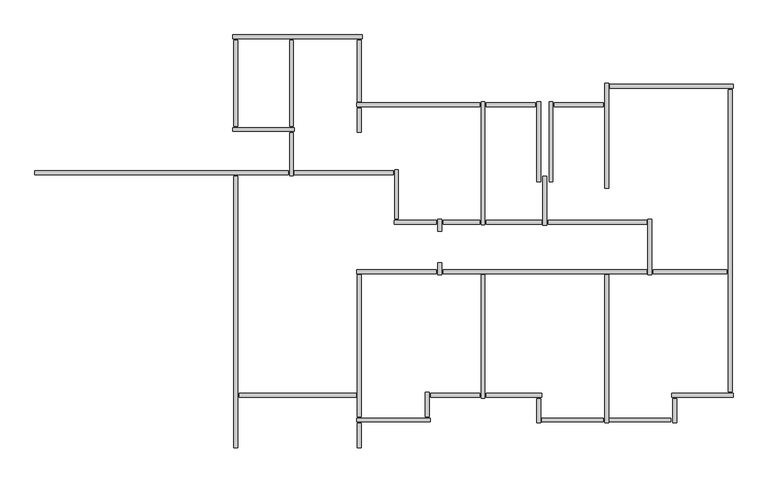
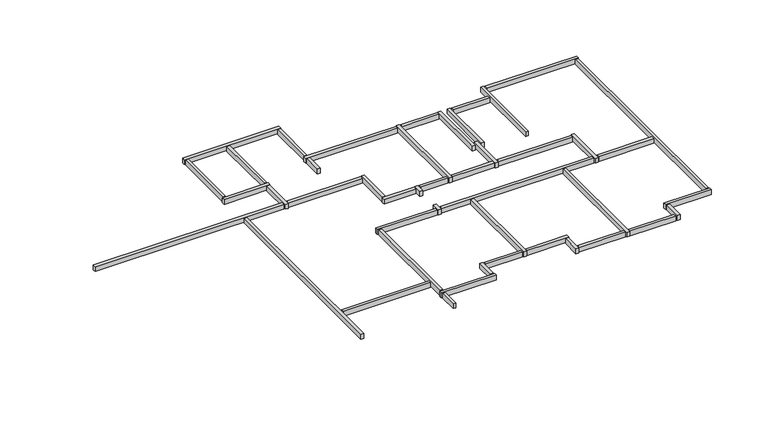
"""IFC4 building model written with IfcOpenShell, lengths in millimetres: beam geometry, Graute viga de respaldo8 : Graute viga de respaldo."""

from ifc_helpers import new_model, si_unit, frame, origin, place, context, project, spatial, polyline, outline, extrude, source, transform, mapped, element, save


def beam_c0cf02b6(model_context):
    return source(origin(), model_context, "Body", "SweptSolid", [
        extrude(outline(polyline([(-54994.9587292, 57408.4278788), (-54994.9587292, 57502.4278788), (-53804.9587292, 57502.4278788), (-53804.9587292, 57408.4278788), (-54994.9587292, 57408.4278788)])), frame((0.0, 0.0, 8632.9999999), z_axis=(0.0, 0.0, 1.0), x_axis=(1.0, 0.0, 0.0)), (0.0, 0.0, 1.0), 167.0),
        extrude(outline(polyline([(-56644.9587292, 57408.4278788), (-56644.9587292, 57502.4278788), (-55454.9587292, 57502.4278788), (-55454.9587292, 57408.4278788), (-56644.9587292, 57408.4278788)])), frame((0.0, 0.0, 8632.9999999), z_axis=(0.0, 0.0, 1.0), x_axis=(1.0, 0.0, 0.0)), (0.0, 0.0, 1.0), 167.0),
        extrude(outline(polyline([(-52594.9587292, 53358.4278788), (-52594.9587292, 53452.4278788), (-50804.9587292, 53452.4278788), (-50804.9587292, 53358.4278788), (-52594.9587292, 53358.4278788)])), frame((0.0, 0.0, 8632.9999999), z_axis=(0.0, 0.0, 1.0), x_axis=(1.0, 0.0, 0.0)), (0.0, 0.0, 1.0), 167.0),
        extrude(outline(polyline([(-57994.9587292, 50358.4278788), (-57994.9587292, 50452.4278788), (-56804.9587292, 50452.4278788), (-56804.9587292, 50358.4278788), (-57994.9587292, 50358.4278788)])), frame((0.0, 0.0, 8632.9999999), z_axis=(0.0, 0.0, 1.0), x_axis=(1.0, 0.0, 0.0)), (0.0, 0.0, 1.0), 167.0),
        extrude(outline(polyline([(-58121.9587292, 50475.4278788), (-58027.9587292, 50475.4278788), (-58027.9587292, 49885.4278788), (-58121.9587292, 49885.4278788), (-58121.9587292, 50475.4278788)])), frame((0.0, 0.0, 8632.9999999), z_axis=(0.0, 0.0, 1.0), x_axis=(1.0, 0.0, 0.0)), (0.0, 0.0, 1.0), 167.0),
        extrude(outline(polyline([(-59794.9587292, 49758.4278788), (-59794.9587292, 49852.4278788), (-58004.9587292, 49852.4278788), (-58004.9587292, 49758.4278788), (-59794.9587292, 49758.4278788)])), frame((0.0, 0.0, 8632.9999999), z_axis=(0.0, 0.0, 1.0), x_axis=(1.0, 0.0, 0.0)), (0.0, 0.0, 1.0), 167.0),
        extrude(outline(polyline([(-57727.9587292, 53335.4278788), (-57821.9587292, 53335.4278788), (-57821.9587292, 53625.4278788), (-57727.9587292, 53625.4278788), (-57727.9587292, 53335.4278788)])), frame((0.0, 0.0, 8632.9999999), z_axis=(0.0, 0.0, 1.0), x_axis=(1.0, 0.0, 0.0)), (0.0, 0.0, 1.0), 167.0),
        extrude(outline(polyline([(-55144.9587292, 54558.4278788), (-55144.9587292, 54652.4278788), (-52754.9587292, 54652.4278788), (-52754.9587292, 54558.4278788), (-55144.9587292, 54558.4278788)])), frame((0.0, 0.0, 8632.9999999), z_axis=(0.0, 0.0, 1.0), x_axis=(1.0, 0.0, 0.0)), (0.0, 0.0, 1.0), 167.0),
        extrude(outline(polyline([(-56644.9587292, 54558.4278788), (-56644.9587292, 54652.4278788), (-55304.9587292, 54652.4278788), (-55304.9587292, 54558.4278788), (-56644.9587292, 54558.4278788)])), frame((0.0, 0.0, 8632.9999999), z_axis=(0.0, 0.0, 1.0), x_axis=(1.0, 0.0, 0.0)), (0.0, 0.0, 1.0), 167.0),
        extrude(outline(polyline([(-57694.9587292, 54558.4278788), (-57694.9587292, 54652.4278788), (-56804.9587292, 54652.4278788), (-56804.9587292, 54558.4278788), (-57694.9587292, 54558.4278788)])), frame((0.0, 0.0, 8632.9999999), z_axis=(0.0, 0.0, 1.0), x_axis=(1.0, 0.0, 0.0)), (0.0, 0.0, 1.0), 167.0),
        extrude(outline(polyline([(-57727.9587292, 54385.4278788), (-57821.9587292, 54385.4278788), (-57821.9587292, 54675.4278788), (-57727.9587292, 54675.4278788), (-57727.9587292, 54385.4278788)])), frame((0.0, 0.0, 8632.9999999), z_axis=(0.0, 0.0, 1.0), x_axis=(1.0, 0.0, 0.0)), (0.0, 0.0, 1.0), 167.0),
        extrude(outline(polyline([(-58884.9587292, 54558.4278788), (-58884.9587292, 54652.4278788), (-57854.9587292, 54652.4278788), (-57854.9587292, 54558.4278788), (-58884.9587292, 54558.4278788)])), frame((0.0, 0.0, 8632.9999999), z_axis=(0.0, 0.0, 1.0), x_axis=(1.0, 0.0, 0.0)), (0.0, 0.0, 1.0), 167.0),
        extrude(outline(polyline([(-58871.9587292, 55875.4278788), (-58777.9587292, 55875.4278788), (-58777.9587292, 54685.4278788), (-58871.9587292, 54685.4278788), (-58871.9587292, 55875.4278788)])), frame((0.0, 0.0, 8632.9999999), z_axis=(0.0, 0.0, 1.0), x_axis=(1.0, 0.0, 0.0)), (0.0, 0.0, 1.0), 167.0),
        extrude(outline(polyline([(-61304.9587292, 55758.4278788), (-61304.9587292, 55852.4278788), (-58904.9587292, 55852.4278788), (-58904.9587292, 55758.4278788), (-61304.9587292, 55758.4278788)])), frame((0.0, 0.0, 8632.9999999), z_axis=(0.0, 0.0, 1.0), x_axis=(1.0, 0.0, 0.0)), (0.0, 0.0, 1.0), 167.0),
        extrude(outline(polyline([(-56677.9587292, 54540.4278788), (-56771.9587292, 54540.4278788), (-56771.9587292, 57525.4278788), (-56677.9587292, 57525.4278788), (-56677.9587292, 54540.4278788)])), frame((0.0, 0.0, 8632.9999999), z_axis=(0.0, 0.0, 1.0), x_axis=(1.0, 0.0, 0.0)), (0.0, 0.0, 1.0), 167.0),
        extrude(outline(polyline([(-59794.9587292, 57408.4278788), (-59794.9587292, 57502.4278788), (-56804.9587292, 57502.4278788), (-56804.9587292, 57408.4278788), (-59794.9587292, 57408.4278788)])), frame((0.0, 0.0, 8632.9999999), z_axis=(0.0, 0.0, 1.0), x_axis=(1.0, 0.0, 0.0)), (0.0, 0.0, 1.0), 167.0),
        extrude(outline(polyline([(-59677.9587292, 56785.4278788), (-59771.9587292, 56785.4278788), (-59771.9587292, 57375.4278788), (-59677.9587292, 57375.4278788), (-59677.9587292, 56785.4278788)])), frame((0.0, 0.0, 8632.9999999), z_axis=(0.0, 0.0, 1.0), x_axis=(1.0, 0.0, 0.0)), (0.0, 0.0, 1.0), 167.0),
        extrude(outline(polyline([(-59771.9587292, 59025.4278788), (-59677.9587292, 59025.4278788), (-59677.9587292, 57535.4278788), (-59771.9587292, 57535.4278788), (-59771.9587292, 59025.4278788)])), frame((0.0, 0.0, 8632.9999999), z_axis=(0.0, 0.0, 1.0), x_axis=(1.0, 0.0, 0.0)), (0.0, 0.0, 1.0), 167.0),
        extrude(outline(polyline([(-62771.9587292, 59025.4278788), (-62677.9587292, 59025.4278788), (-62677.9587292, 56935.4278788), (-62771.9587292, 56935.4278788), (-62771.9587292, 59025.4278788)])), frame((0.0, 0.0, 8632.9999999), z_axis=(0.0, 0.0, 1.0), x_axis=(1.0, 0.0, 0.0)), (0.0, 0.0, 1.0), 167.0),
        extrude(outline(polyline([(-61421.9587292, 59025.4278788), (-61327.9587292, 59025.4278788), (-61327.9587292, 56935.4278788), (-61421.9587292, 56935.4278788), (-61421.9587292, 59025.4278788)])), frame((0.0, 0.0, 8632.9999999), z_axis=(0.0, 0.0, 1.0), x_axis=(1.0, 0.0, 0.0)), (0.0, 0.0, 1.0), 167.0),
        extrude(outline(polyline([(-61327.9587292, 55735.4278788), (-61421.9587292, 55735.4278788), (-61421.9587292, 56775.4278788), (-61327.9587292, 56775.4278788), (-61327.9587292, 55735.4278788)])), frame((0.0, 0.0, 8632.9999999), z_axis=(0.0, 0.0, 1.0), x_axis=(1.0, 0.0, 0.0)), (0.0, 0.0, 1.0), 167.0),
        extrude(outline(polyline([(-62644.9587292, 50358.4278788), (-62644.9587292, 50452.4278788), (-59804.9587292, 50452.4278788), (-59804.9587292, 50358.4278788), (-62644.9587292, 50358.4278788)])), frame((0.0, 0.0, 8632.9999999), z_axis=(0.0, 0.0, 1.0), x_axis=(1.0, 0.0, 0.0)), (0.0, 0.0, 1.0), 167.0),
        extrude(outline(polyline([(-59771.9587292, 53325.4278788), (-59677.9587292, 53325.4278788), (-59677.9587292, 49885.4278788), (-59771.9587292, 49885.4278788), (-59771.9587292, 53325.4278788)])), frame((0.0, 0.0, 8632.9999999), z_axis=(0.0, 0.0, 1.0), x_axis=(1.0, 0.0, 0.0)), (0.0, 0.0, 1.0), 167.0),
        extrude(outline(polyline([(-59794.9587292, 53358.4278788), (-59794.9587292, 53452.4278788), (-57854.9587292, 53452.4278788), (-57854.9587292, 53358.4278788), (-59794.9587292, 53358.4278788)])), frame((0.0, 0.0, 8632.9999999), z_axis=(0.0, 0.0, 1.0), x_axis=(1.0, 0.0, 0.0)), (0.0, 0.0, 1.0), 167.0),
        extrude(outline(polyline([(-57694.9587292, 53358.4278788), (-57694.9587292, 53452.4278788), (-52754.9587292, 53452.4278788), (-52754.9587292, 53358.4278788), (-57694.9587292, 53358.4278788)])), frame((0.0, 0.0, 8632.9999999), z_axis=(0.0, 0.0, 1.0), x_axis=(1.0, 0.0, 0.0)), (0.0, 0.0, 1.0), 167.0),
        extrude(outline(polyline([(-56677.9587292, 50335.4278788), (-56771.9587292, 50335.4278788), (-56771.9587292, 53325.4278788), (-56677.9587292, 53325.4278788), (-56677.9587292, 50335.4278788)])), frame((0.0, 0.0, 8632.9999999), z_axis=(0.0, 0.0, 1.0), x_axis=(1.0, 0.0, 0.0)), (0.0, 0.0, 1.0), 167.0),
        extrude(outline(polyline([(-55304.9587292, 50452.4278788), (-55304.9587292, 50358.4278788), (-56644.9587292, 50358.4278788), (-56644.9587292, 50452.4278788), (-55304.9587292, 50452.4278788)])), frame((0.0, 0.0, 8632.9999999), z_axis=(0.0, 0.0, 1.0), x_axis=(1.0, 0.0, 0.0)), (0.0, 0.0, 1.0), 167.0),
        extrude(outline(polyline([(-55327.9587292, 49735.4278788), (-55421.9587292, 49735.4278788), (-55421.9587292, 50325.4278788), (-55327.9587292, 50325.4278788), (-55327.9587292, 49735.4278788)])), frame((0.0, 0.0, 8632.9999999), z_axis=(0.0, 0.0, 1.0), x_axis=(1.0, 0.0, 0.0)), (0.0, 0.0, 1.0), 167.0),
        extrude(outline(polyline([(-55294.9587292, 49758.4278788), (-55294.9587292, 49852.4278788), (-53804.9587292, 49852.4278788), (-53804.9587292, 49758.4278788), (-55294.9587292, 49758.4278788)])), frame((0.0, 0.0, 8632.9999999), z_axis=(0.0, 0.0, 1.0), x_axis=(1.0, 0.0, 0.0)), (0.0, 0.0, 1.0), 167.0),
        extrude(outline(polyline([(-52165.9809043, 49853.4278788), (-52165.9809043, 49758.4278788), (-53654.9587292, 49758.4278788), (-53654.9587292, 49853.4278788), (-52165.9809043, 49853.4278788)])), frame((0.0, 0.0, 8617.1856208), z_axis=(0.0, 0.0, 1.0), x_axis=(1.0, 0.0, 0.0)), (0.0, 0.0, 1.0), 165.0),
        extrude(outline(polyline([(-50771.9587292, 57825.4278788), (-50677.9587292, 57825.4278788), (-50677.9587292, 50485.4278788), (-50771.9587292, 50485.4278788), (-50771.9587292, 57825.4278788)])), frame((0.0, 0.0, 8632.9999999), z_axis=(0.0, 0.0, 1.0), x_axis=(1.0, 0.0, 0.0)), (0.0, 0.0, 1.0), 167.0),
        extrude(outline(polyline([(-52721.9587292, 54675.4278788), (-52627.9587292, 54675.4278788), (-52627.9587292, 53330.0746661), (-52721.9587292, 53330.0746661), (-52721.9587292, 54675.4278788)])), frame((0.0, 0.0, 8632.9999999), z_axis=(0.0, 0.0, 1.0), x_axis=(1.0, 0.0, 0.0)), (0.0, 0.0, 1.0), 167.0),
        extrude(outline(polyline([(-55271.9587292, 55725.4278788), (-55177.9587292, 55725.4278788), (-55177.9587292, 54535.4278788), (-55271.9587292, 54535.4278788), (-55271.9587292, 55725.4278788)])), frame((0.0, 0.0, 8632.9999999), z_axis=(0.0, 0.0, 1.0), x_axis=(1.0, 0.0, 0.0)), (0.0, 0.0, 1.0), 167.0),
        extrude(outline(polyline([(-55121.9587292, 57525.4278788), (-55027.9587292, 57525.4278788), (-55027.9587292, 55585.4278788), (-55121.9587292, 55585.4278788), (-55121.9587292, 57525.4278788)])), frame((0.0, 0.0, 8632.9999999), z_axis=(0.0, 0.0, 1.0), x_axis=(1.0, 0.0, 0.0)), (0.0, 0.0, 1.0), 167.0),
        extrude(outline(polyline([(-55421.9587292, 57525.4278788), (-55327.9587292, 57525.4278788), (-55327.9587292, 55585.4278788), (-55421.9587292, 55585.4278788), (-55421.9587292, 57525.4278788)])), frame((0.0, 0.0, 8632.9999999), z_axis=(0.0, 0.0, 1.0), x_axis=(1.0, 0.0, 0.0)), (0.0, 0.0, 1.0), 167.0),
        extrude(outline(polyline([(-53771.9587292, 57975.4278788), (-53677.9587292, 57975.4278788), (-53677.9587292, 55435.4278788), (-53771.9587292, 55435.4278788), (-53771.9587292, 57975.4278788)])), frame((0.0, 0.0, 8632.9999999), z_axis=(0.0, 0.0, 1.0), x_axis=(1.0, 0.0, 0.0)), (0.0, 0.0, 1.0), 167.0),
        extrude(outline(polyline([(-50654.9587292, 57952.4278788), (-50654.9587292, 57858.4278788), (-53644.9587292, 57858.4278788), (-53644.9587292, 57952.4278788), (-50654.9587292, 57952.4278788)])), frame((0.0, 0.0, 8632.9999999), z_axis=(0.0, 0.0, 1.0), x_axis=(1.0, 0.0, 0.0)), (0.0, 0.0, 1.0), 167.0),
        extrude(outline(polyline([(-52027.9587292, 49735.4278788), (-52121.9587292, 49735.4278788), (-52121.9587292, 50325.4278788), (-52027.9587292, 50325.4278788), (-52027.9587292, 49735.4278788)])), frame((0.0, 0.0, 8632.9999999), z_axis=(0.0, 0.0, 1.0), x_axis=(1.0, 0.0, 0.0)), (0.0, 0.0, 1.0), 167.0),
        extrude(outline(polyline([(-52144.9587292, 50358.4278788), (-52144.9587292, 50452.4278788), (-50654.9587292, 50452.4278788), (-50654.9587292, 50358.4278788), (-52144.9587292, 50358.4278788)])), frame((0.0, 0.0, 8632.9999999), z_axis=(0.0, 0.0, 1.0), x_axis=(1.0, 0.0, 0.0)), (0.0, 0.0, 1.0), 167.0),
        extrude(outline(polyline([(-53677.9587292, 49735.4278788), (-53771.9587292, 49735.4278788), (-53771.9587292, 53325.4278788), (-53677.9587292, 53325.4278788), (-53677.9587292, 49735.4278788)])), frame((0.0, 0.0, 8632.9999999), z_axis=(0.0, 0.0, 1.0), x_axis=(1.0, 0.0, 0.0)), (0.0, 0.0, 1.0), 167.0),
        extrude(outline(polyline([(-59677.9587292, 49135.4278788), (-59771.9587292, 49135.4278788), (-59771.9587292, 49725.4278788), (-59677.9587292, 49725.4278788), (-59677.9587292, 49135.4278788)])), frame((0.0, 0.0, 8632.9999999), z_axis=(0.0, 0.0, 1.0), x_axis=(1.0, 0.0, 0.0)), (0.0, 0.0, 1.0), 167.0),
        extrude(outline(polyline([(-62794.9587292, 56808.4278788), (-62794.9587292, 56902.4278788), (-61304.9587292, 56902.4278788), (-61304.9587292, 56808.4278788), (-62794.9587292, 56808.4278788)])), frame((0.0, 0.0, 8632.9999999), z_axis=(0.0, 0.0, 1.0), x_axis=(1.0, 0.0, 0.0)), (0.0, 0.0, 1.0), 167.0),
        extrude(outline(polyline([(-62794.9587292, 59058.4278788), (-62794.9587292, 59152.4278788), (-59654.9587292, 59152.4278788), (-59654.9587292, 59058.4278788), (-62794.9587292, 59058.4278788)])), frame((0.0, 0.0, 8632.9999999), z_axis=(0.0, 0.0, 1.0), x_axis=(1.0, 0.0, 0.0)), (0.0, 0.0, 1.0), 167.0),
        extrude(outline(polyline([(-67601.7587292, 55758.4278788), (-67601.7587292, 55852.4278788), (-61454.9587292, 55852.4278788), (-61454.9587292, 55758.4278788), (-67601.7587292, 55758.4278788)])), frame((0.0, 0.0, 8632.9999999), z_axis=(0.0, 0.0, 1.0), x_axis=(1.0, 0.0, 0.0)), (0.0, 0.0, 1.0), 167.0),
        extrude(outline(polyline([(-62677.9587292, 49132.8979841), (-62771.9587292, 49132.8979841), (-62771.9587292, 55725.4278788), (-62677.9587292, 55725.4278788), (-62677.9587292, 49132.8979841)])), frame((0.0, 0.0, 8632.9999999), z_axis=(0.0, 0.0, 1.0), x_axis=(1.0, 0.0, 0.0)), (0.0, 0.0, 1.0), 167.0),
    ])


if __name__ == "__main__":
    model = new_model("IFC4")
    model_context = context("Model", 3, world=origin())
    ifc_project = project(units=[si_unit("LENGTHUNIT", "METRE", prefix="MILLI")], contexts=[model_context])
    site = spatial("IfcSite", under=ifc_project)
    building = spatial("IfcBuilding", under=site)
    placement = place(None, origin())
    beam_shape = beam_c0cf02b6(model_context)
    element("IfcBeam", 1, ObjectType="Graute viga de respaldo8 : Graute viga de respaldo", at=placement, inside=building, context=model_context, shape_type="MappedRepresentation", body=[
        mapped(beam_shape, transform((0.0, 0.0, 0.0), x_axis=(1.0, 0.0, 0.0), y_axis=(0.0, 1.0, 0.0), z_axis=(0.0, 0.0, 1.0))),
    ])
    save(model, "model.ifc")

# Revit data of these elements
# Element 1 (IfcBeam, "Graute viga de respaldo8 : Graute viga de respaldo")
#   Materials on its faces: "Concreto, Faixa de areia/cimento"
# Materials
#   "Concreto, Faixa de areia/cimento": class "Concreto", colour RGB 127 127 127, transparency 0, Description = "Revestimento de laje de concreto", Cost = 0
